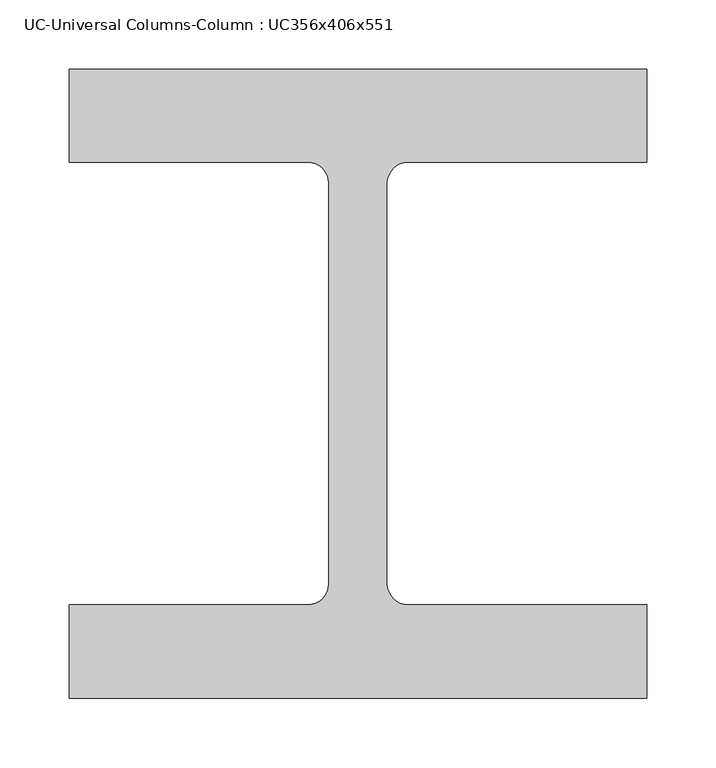
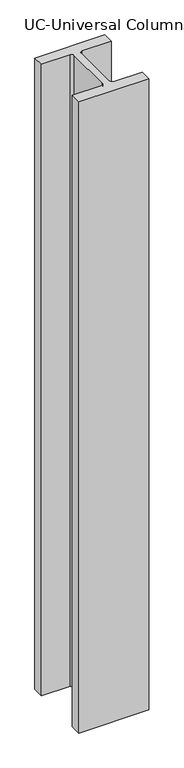
"""IFC4 building model written with IfcOpenShell, lengths in millimetres: column geometry, UC-Universal Columns-Column : UC356x406x551."""

from ifc_helpers import new_model, si_unit, point, frame, frame_2d, origin, place, context, project, spatial, polyline, circle_curve, trimmed, segment, composite_curve, outline, extrude, source, transform, mapped, element, save


def uc_universal_columns_column_uc356x406x551_decfc3ec(model_context):
    return source(origin(), model_context, "Body", "SweptSolid", [
        extrude(outline(composite_curve([segment(polyline([(209.25, 227.8), (209.25, 160.3), (36.25, 160.3)]), True, "CONTINUOUS"), segment(trimmed(circle_curve(frame_2d((36.25, 145.1)), 15.2), [point((36.25, 160.3))], [point((21.05, 145.1))], True, "CARTESIAN"), True, "CONTINUOUS"), segment(polyline([(21.05, 145.1), (21.05, -145.1)]), True, "CONTINUOUS"), segment(trimmed(circle_curve(frame_2d((36.25, -145.1)), 15.2), [point((21.05, -145.1))], [point((36.25, -160.3))], True, "CARTESIAN"), True, "CONTINUOUS"), segment(polyline([(36.25, -160.3), (209.25, -160.3), (209.25, -227.8), (-209.25, -227.8), (-209.25, -160.3), (-36.25, -160.3)]), True, "CONTINUOUS"), segment(trimmed(circle_curve(frame_2d((-36.25, -145.1)), 15.2), [point((-36.25, -160.3))], [point((-21.05, -145.1))], True, "CARTESIAN"), True, "CONTINUOUS"), segment(polyline([(-21.05, -145.1), (-21.05, 145.1)]), True, "CONTINUOUS"), segment(trimmed(circle_curve(frame_2d((-36.25, 145.1)), 15.2), [point((-21.05, 145.1))], [point((-36.25, 160.3))], True, "CARTESIAN"), True, "CONTINUOUS"), segment(polyline([(-36.25, 160.3), (-209.25, 160.3), (-209.25, 227.8), (209.25, 227.8)]), True, "CONTINUOUS")], self_intersect=False)), frame((0.0, 0.0, 4000.0), z_axis=(0.0, 0.0, 1.0), x_axis=(1.0, 0.0, 0.0)), (0.0, 0.0, 1.0), 4000.0),
    ])


if __name__ == "__main__":
    model = new_model("IFC4")
    model_context = context("Model", 3, world=origin())
    ifc_project = project(units=[si_unit("LENGTHUNIT", "METRE", prefix="MILLI")], contexts=[model_context])
    site = spatial("IfcSite", under=ifc_project)
    building = spatial("IfcBuilding", under=site)
    placement = place(None, origin())
    uc_universal_columns_column_uc356x406x551_shape = uc_universal_columns_column_uc356x406x551_decfc3ec(model_context)
    element("IfcColumn", 1, ObjectType="UC-Universal Columns-Column : UC356x406x551", at=placement, inside=building, context=model_context, shape_type="MappedRepresentation", body=[
        mapped(uc_universal_columns_column_uc356x406x551_shape, transform((0.0, 0.0, 0.0), x_axis=(1.0, 0.0, 0.0), y_axis=(0.0, 1.0, 0.0), z_axis=(0.0, 0.0, 1.0))),
    ])
    save(model, "model.ifc")

# Revit data of these elements
# Type "UC-Universal Columns-Column : UC356x406x551"
#   Section Name Key = "UC356x406x551"
#   Width = 41.85 cm
#   Web Thickness = 4.21 cm
#   Web Fillet = 1.52 cm
#   Warping Constant = 31100000.0 cm⁶
#   Torsional Moment of Inertia = 9240.00 cm⁴
#   Section Area = 702.0 cm²
#   Plastic Modulus weak axis = 6058.0 cm³
#   Plastic Modulus strong axis = 12076.0 cm³
#   Nominal Weight = 551.00 kgf/m
#   Moment of Inertia weak axis = 82671.00 cm⁴
#   Moment of Inertia strong axis = 226938.00 cm⁴
#   Height = 45.56 cm
#   Flange Thickness = 6.75 cm
#   Elastic Modulus weak axis = 3951.0 cm³
#   Elastic Modulus strong axis = 9962.0 cm³
#   Centroid Vertical = 22.78 cm
#   Centroid Horizontal = 20.925 cm
#   built-in parameter 1005541 = 0.246063 (stored number, unit not read)
#   built-in parameter 1005540 = 0.459318 (stored number, unit not read)
#   Bolt Spacing = 14.0 cm
#   Structural Material [instance default] = Metal - Steel 43-275
#   Type Comments = ""
#   Assembly Code = ""
# Element 1 (IfcColumn, "UC-Universal Columns-Column : UC356x406x551")
#   Materials on its faces: "Metal - Steel 43-275"
# Materials
#   "Metal - Steel 43-275": class "Metal", colour RGB 247 247 247, transparency 0, Cost = 0
